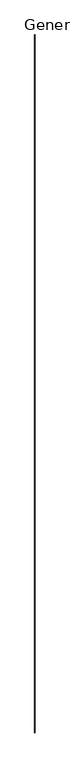
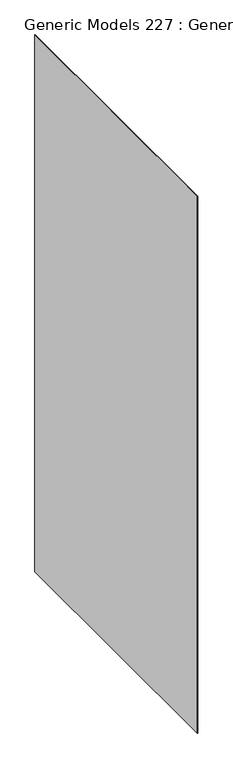
"""IFC4 building model written with IfcOpenShell, lengths in millimetres: proxy geometry, Generic Models 227 : Generic Models 46."""

from ifc_helpers import new_model, si_unit, frame, origin, place, context, project, spatial, polyline, outline, extrude, source, transform, mapped, element, save


def generic_models_227_generic_models_46_e0d4e21f(model_context):
    return source(origin(), model_context, "Body", "SweptSolid", [
        extrude(outline(polyline([(48566.0211605, 0.0), (48565.2274105, 0.0), (48565.2274105, 1219.2), (48566.0211605, 1219.2), (48566.0211605, 0.0)])), frame((0.0, 0.0, 3049.1358009), z_axis=(0.0, 0.0, 1.0), x_axis=(1.0, 0.0, 0.0)), (0.0, 0.0, 1.0), 2456.7781344),
    ])


if __name__ == "__main__":
    model = new_model("IFC4")
    model_context = context("Model", 3, world=origin())
    ifc_project = project(units=[si_unit("LENGTHUNIT", "METRE", prefix="MILLI")], contexts=[model_context])
    site = spatial("IfcSite", under=ifc_project)
    building = spatial("IfcBuilding", under=site)
    placement = place(None, origin())
    generic_models_227_generic_models_46_shape = generic_models_227_generic_models_46_e0d4e21f(model_context)
    element("IfcBuildingElementProxy", 1, Name="Generic Models 227 : Generic Models 46", ObjectType="Generic Models 227 : Generic Models 46", at=placement, inside=building, context=model_context, shape_type="MappedRepresentation", body=[
        mapped(generic_models_227_generic_models_46_shape, transform((0.0, 0.0, 0.0), x_axis=(1.0, 0.0, 0.0), y_axis=(0.0, 1.0, 0.0), z_axis=(0.0, 0.0, 1.0))),
    ])
    save(model, "model.ifc")

# Revit data of these elements
# Element 1 (IfcBuildingElementProxy, "Generic Models 227 : Generic Models 46")
#   Materials on its faces: "6 MIL VAPOR BARRIER"
# Materials
#   "6 MIL VAPOR BARRIER": class "Generic", colour RGB 66 158 52, transparency 0, Cost = 0
